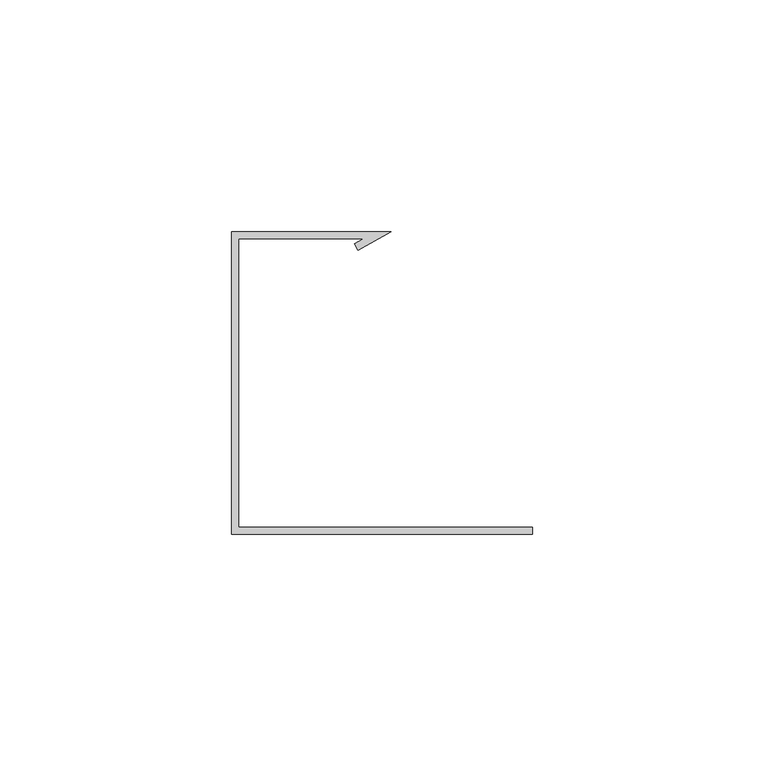
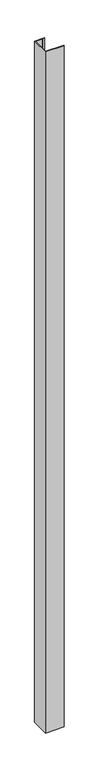
"""IFC4 building model written with IfcOpenShell, lengths in millimetres: proxy geometry, Generic Models 2:Generic Models 2:310765:Generic Models 2:310765 : Generic Models 2:Generic Models 2:310765:85 : Generic Models 2:Generic Models 2:310765:Generic Models 2:310765 : Generic Models 2:Generic Models 2:310765:300385."""

import ifcopenshell
import ifcopenshell.guid

model = None  # the IFC model being written
_history = None  # IfcOwnerHistory: only IFC2X3 demands one
_inside = {}  # id of a spatial element -> (the spatial element, [elements in it])
_under = {}  # id of a project, library or spatial element -> (it, [spatial elements below it])
_declared = {}  # id of a project -> (the project, [libraries it declares])
_typed = {}  # id of a type object -> (the type object, [elements of that type])
_made_of = {}  # id of a material, layer set ... -> (it, [elements and type objects made of it])


def new_model(schema):
    """Start an empty IFC model of exactly this schema.

    Asked for "IFC4X3", IfcOpenShell would pick the latest addendum, in which some entities
    have other attributes; the version numbers below select the first issue.
    IFC2X3 requires an IfcOwnerHistory on every rooted entity: one is made here for all.
    """
    global model, _history
    if schema == "IFC4X3":
        model = ifcopenshell.file(schema_version=(4, 3, 0, 0))
    else:
        model = ifcopenshell.file(schema=schema)
    _inside.clear()
    _under.clear()
    _declared.clear()
    _typed.clear()
    _made_of.clear()
    _history = None
    if model.schema == "IFC2X3":
        org = make("IfcOrganization", Name="unknown")
        user = make(
            "IfcPersonAndOrganization",
            ThePerson=make("IfcPerson", FamilyName="unknown"),
            TheOrganization=org,
        )
        app = make(
            "IfcApplication",
            ApplicationDeveloper=org,
            Version="unknown",
            ApplicationFullName="unknown",
            ApplicationIdentifier="unknown",
        )
        _history = make(
            "IfcOwnerHistory",
            OwningUser=user,
            OwningApplication=app,
            ChangeAction="ADDED",
            CreationDate=0,
        )
    return model


def make(cls, **values):
    """One entity of the class cls with the attributes given. An attribute that is None is left unset."""
    return model.create_entity(
        cls, **{name: value for name, value in values.items() if value is not None}
    )


def rooted(cls, **values):
    """An entity with a GlobalId (a new one), such as an element, a storey or a relation."""
    return make(cls, GlobalId=ifcopenshell.guid.new(), OwnerHistory=_history, **values)


def si_unit(unit_type, name, prefix=None):
    """IfcSIUnit, for example si_unit("LENGTHUNIT", "METRE", prefix="MILLI")."""
    return make("IfcSIUnit", UnitType=unit_type, Prefix=prefix, Name=name)


def assignment(units):
    """IfcUnitAssignment: the units of a project."""
    return None if units is None else make("IfcUnitAssignment", Units=units)


def point(xyz):
    """IfcCartesianPoint."""
    return None if xyz is None else make("IfcCartesianPoint", Coordinates=xyz)


def direction(xyz):
    """IfcDirection."""
    return None if xyz is None else make("IfcDirection", DirectionRatios=xyz)


def frame(location, z_axis=None, x_axis=None):
    """IfcAxis2Placement3D, a coordinate frame: its origin and axes. An axis left out is left unset."""
    return make(
        "IfcAxis2Placement3D",
        Location=point(location),
        Axis=direction(z_axis),
        RefDirection=direction(x_axis),
    )


def origin():
    """The frame at (0, 0, 0) with its axes left unset."""
    return frame((0.0, 0.0, 0.0))


def origin_with_axes():
    """The frame at (0, 0, 0) with the z axis (0, 0, 1) and the x axis (1, 0, 0) written out."""
    return frame((0.0, 0.0, 0.0), z_axis=(0.0, 0.0, 1.0), x_axis=(1.0, 0.0, 0.0))


def place(relative_to, where):
    """IfcLocalPlacement: puts the frame where relative to a parent placement (None: the world)."""
    return make(
        "IfcLocalPlacement", PlacementRelTo=relative_to, RelativePlacement=where
    )


def context(
    kind, dimensions, precision=None, world=None, true_north=None, identifier=None
):
    """IfcGeometricRepresentationContext, for example the 3D "Model" context."""
    return make(
        "IfcGeometricRepresentationContext",
        ContextIdentifier=identifier,
        ContextType=kind,
        CoordinateSpaceDimension=dimensions,
        Precision=precision,
        WorldCoordinateSystem=world,
        TrueNorth=true_north,
    )


def project(units=None, contexts=None):
    """IfcProject with its units and contexts."""
    return rooted(
        "IfcProject",
        Name="project",
        RepresentationContexts=contexts,
        UnitsInContext=assignment(units),
    )


def spatial(cls, under=None, at=None, **own):
    """A site, building, storey or space (cls), placed at a placement, below another one or the project."""
    s = rooted(cls, ObjectPlacement=at, **own)
    if under is not None:
        _under.setdefault(under.id(), (under, []))[1].append(s)
    return s


def polyline(points):
    """IfcPolyline through the points."""
    return make("IfcPolyline", Points=[point(p) for p in points])


def outline(outer, holes=None, kind="AREA"):
    """IfcArbitraryClosedProfileDef: a profile drawn as a closed curve; with holes, ...WithVoids."""
    if holes is None:
        return make("IfcArbitraryClosedProfileDef", ProfileType=kind, OuterCurve=outer)
    return make(
        "IfcArbitraryProfileDefWithVoids",
        ProfileType=kind,
        OuterCurve=outer,
        InnerCurves=holes,
    )


def extrude(swept, where, along, depth):
    """IfcExtrudedAreaSolid: the profile swept, set in the frame where, extruded along a direction by depth."""
    return make(
        "IfcExtrudedAreaSolid",
        SweptArea=swept,
        Position=where,
        ExtrudedDirection=direction(along),
        Depth=depth,
    )


def shape(context_of_items, identifier, shape_type, items):
    """IfcShapeRepresentation: the items that make up one representation, for example the "Body"."""
    return make(
        "IfcShapeRepresentation",
        ContextOfItems=context_of_items,
        RepresentationIdentifier=identifier,
        RepresentationType=shape_type,
        Items=items,
    )


def source(mapping_origin, context_of_items, identifier, shape_type, items):
    """IfcRepresentationMap: a shape defined once, which mapped items show again and again."""
    return make(
        "IfcRepresentationMap",
        MappingOrigin=mapping_origin,
        MappedRepresentation=shape(context_of_items, identifier, shape_type, items),
    )


def transform(
    local_origin,
    x_axis=None,
    y_axis=None,
    z_axis=None,
    scale=None,
    scale2=None,
    scale3=None,
    uniform=True,
):
    """IfcCartesianTransformationOperator3D, or its non-uniform kind. x_axis, y_axis, z_axis: its Axis1, 2, 3."""
    if uniform:
        return make(
            "IfcCartesianTransformationOperator3D",
            Axis1=direction(x_axis),
            Axis2=direction(y_axis),
            LocalOrigin=point(local_origin),
            Scale=scale,
            Axis3=direction(z_axis),
        )
    return make(
        "IfcCartesianTransformationOperator3DnonUniform",
        Axis1=direction(x_axis),
        Axis2=direction(y_axis),
        LocalOrigin=point(local_origin),
        Scale=scale,
        Axis3=direction(z_axis),
        Scale2=scale2,
        Scale3=scale3,
    )


def mapped(mapping_source, mapping_target):
    """IfcMappedItem: shows the shape of a source again, moved by a transform."""
    return make(
        "IfcMappedItem", MappingSource=mapping_source, MappingTarget=mapping_target
    )


def made_of(thing, what):
    """Note that an element or type object is made of a material, layer set ...; save() writes the relation."""
    if what is not None:
        _made_of.setdefault(what.id(), (what, []))[1].append(thing)
    return thing


def element(
    cls,
    number,
    at=None,
    inside=None,
    cuts=None,
    type_object=None,
    material=None,
    context=None,
    identifier="Body",
    shape_type=None,
    held_by="IfcProductDefinitionShape",
    body=None,
    shapes=None,
    **own,
):
    """One element of the class cls, such as IfcWall. Its Tag is "e" and its number.

    at: its placement. inside: the storey or other place that contains it. cuts: it is an
    opening in that element (IfcRelVoidsElement). A single representation is given by context,
    identifier, shape_type and body (its items); several are given by shapes. held_by: the class
    of the entity that holds the representations. save() writes the other relations.
    """
    e = rooted(cls, Tag="e%d" % number, ObjectPlacement=at, **own)
    if body is not None:
        shapes = [shape(context, identifier, shape_type, body)]
    if shapes is not None:
        e.Representation = make(held_by, Representations=shapes)
    if inside is not None:
        _inside.setdefault(inside.id(), (inside, []))[1].append(e)
    if cuts is not None:
        rooted(
            "IfcRelVoidsElement", RelatingBuildingElement=cuts, RelatedOpeningElement=e
        )
    if type_object is not None:
        _typed.setdefault(type_object.id(), (type_object, []))[1].append(e)
    return made_of(e, material)


def aggregate(whole, parts):
    """IfcRelAggregates: a whole, such as a stair, and the parts it consists of."""
    return rooted("IfcRelAggregates", RelatingObject=whole, RelatedObjects=parts)


def save(model, path):
    """Write the relations noted so far, then the file.

    IfcRelAggregates (storeys below a building ...), IfcRelContainedInSpatialStructure (elements
    in a storey), IfcRelDefinesByType, IfcRelAssociatesMaterial and IfcRelDeclares: one each for
    every whole, place, type object, material and project.
    """
    for whole, parts in _under.values():
        aggregate(whole, parts)
    for where, things in _inside.values():
        rooted(
            "IfcRelContainedInSpatialStructure",
            RelatedElements=things,
            RelatingStructure=where,
        )
    for kind, things in _typed.values():
        rooted("IfcRelDefinesByType", RelatedObjects=things, RelatingType=kind)
    for what, things in _made_of.values():
        rooted("IfcRelAssociatesMaterial", RelatedObjects=things, RelatingMaterial=what)
    for by, libraries in _declared.values():
        rooted("IfcRelDeclares", RelatingContext=by, RelatedDefinitions=libraries)
    model.write(path)


def generic_models_d22cce78(model_context):
    return source(origin(), model_context, "Body", "SweptSolid", [
        extrude(outline(polyline([(593781.8548288, -536555.276206), (593781.8548288, -536489.8453125), (593816.3294723, -536489.8453125), (593809.2756123, -536493.9178604), (593808.4818623, -536492.5430451), (593810.4048416, -536491.4328125), (593783.4423288, -536491.4328125), (593783.4423288, -536553.688706), (593846.9423288, -536553.688706), (593846.9423288, -536555.276206), (593781.8548288, -536555.276206)])), origin_with_axes(), (0.0, 0.0, 1.0), 2508.9309299),
    ])


if __name__ == "__main__":
    model = new_model("IFC4")
    model_context = context("Model", 3, world=origin())
    ifc_project = project(units=[si_unit("LENGTHUNIT", "METRE", prefix="MILLI")], contexts=[model_context])
    site = spatial("IfcSite", under=ifc_project)
    building = spatial("IfcBuilding", under=site)
    placement = place(None, origin())
    generic_models_shape = generic_models_d22cce78(model_context)
    element("IfcBuildingElementProxy", 1, Name="Generic Models 2:Generic Models 2:310765:Generic Models 2:310765 : Generic Models 2:Generic Models 2:310765:85 : Generic Models 2:Generic Models 2:310765:Generic Models 2:310765 : Generic Models 2:Generic Models 2:310765:300385", ObjectType="Generic Models 2:Generic Models 2:310765:Generic Models 2:310765 : Generic Models 2:Generic Models 2:310765:85 : Generic Models 2:Generic Models 2:310765:Generic Models 2:310765 : Generic Models 2:Generic Models 2:310765:300385", at=placement, inside=building, context=model_context, shape_type="MappedRepresentation", body=[
        mapped(generic_models_shape, transform((0.0, 0.0, 0.0), x_axis=(1.0, 0.0, 0.0), y_axis=(0.0, 1.0, 0.0), z_axis=(0.0, 0.0, 1.0))),
    ])
    save(model, "model.ifc")

# Revit data of these elements
# Type "Generic Models 2:Generic Models 2:310765:Generic Models 2:310765 : Generic Models 2:Generic Models 2:310765:85 : Generic Models 2:Generic Models 2:310765:Generic Models 2:310765 : Generic Models 2:Generic Models 2:310765:300385"
#   NameOverride = "Generic Models 2:Generic Models 2:310765:Generic Models 2:310765 : Generic Models 2:Generic Models 2:310765:300385"
#   ObjectTypeOverride = "Generic Models 2:310765 : Generic Models 2:Generic Models 2:310765"
#   Reference = "Generic Models 2"
#   Tag = "300385"
# Element 1 (IfcBuildingElementProxy, "Generic Models 2:Generic Models 2:310765:Generic Models 2:310765 : Generic Models 2:Generic Models 2:310765:85 : Generic Models 2:Generic Models 2:310765:Generic Models 2:310765 : Generic Models 2:Generic Models 2:310765:300385")
#   Materials on its faces: "JAMB TRIM"
# Materials
#   "JAMB TRIM": class "Unassigned", colour RGB 210 209 208, transparency 0, Cost = 0
